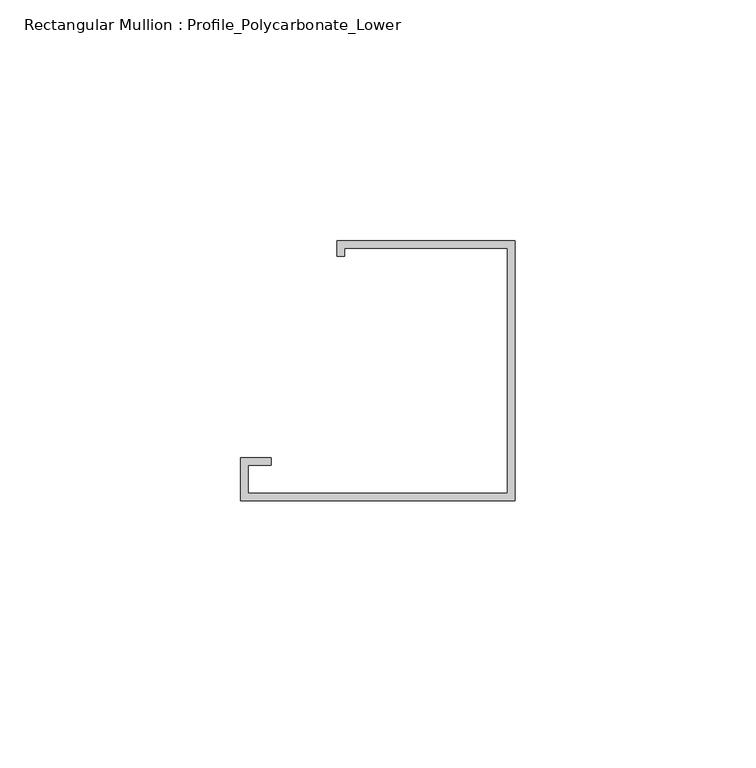
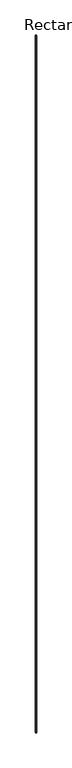
"""IFC4 building model written with IfcOpenShell, lengths in millimetres: member geometry, Rectangular Mullion : Profile_Polycarbonate_Lower."""

from ifc_helpers import new_model, si_unit, frame, origin, place, context, project, spatial, polyline, outline, extrude, source, transform, mapped, element, save


def rectangular_mullion_profile_polycarbonate_lower_9942ed0a(model_context):
    return source(origin(), model_context, "Body", "SweptSolid", [
        extrude(outline(polyline([(0.0, -28.984575), (-56.9976, -28.984575), (-56.9976, -19.992975), (-50.6476, -19.992975), (-50.6476, -21.580475), (-55.4101, -21.580475), (-55.4101, -27.397075), (-1.5875, -27.397075), (-1.5875, 23.428325), (-35.3949, 23.428325), (-35.3949, 21.840825), (-36.9824, 21.840825), (-36.9824, 25.015825), (0.0, 25.015825), (0.0, -28.984575)])), frame((0.0, 0.0, -31440.30288), z_axis=(0.0, 0.0, 1.0), x_axis=(1.0, 0.0, 0.0)), (0.0, 0.0, 1.0), 31440.30288),
    ])


if __name__ == "__main__":
    model = new_model("IFC4")
    model_context = context("Model", 3, world=origin())
    ifc_project = project(units=[si_unit("LENGTHUNIT", "METRE", prefix="MILLI")], contexts=[model_context])
    site = spatial("IfcSite", under=ifc_project)
    building = spatial("IfcBuilding", under=site)
    placement = place(None, origin())
    rectangular_mullion_profile_polycarbonate_lower_shape = rectangular_mullion_profile_polycarbonate_lower_9942ed0a(model_context)
    element("IfcMember", 1, ObjectType="Rectangular Mullion : Profile_Polycarbonate_Lower", at=placement, inside=building, context=model_context, shape_type="MappedRepresentation", body=[
        mapped(rectangular_mullion_profile_polycarbonate_lower_shape, transform((0.0, 0.0, 0.0), x_axis=(1.0, 0.0, 0.0), y_axis=(0.0, 1.0, 0.0), z_axis=(0.0, 0.0, 1.0))),
    ])
    save(model, "model.ifc")

# Revit data of these elements
# Type "Rectangular Mullion : Profile_Polycarbonate_Lower"
#   built-in parameter 1007322 = 0.177167 (stored number, unit not read)
#   built-in parameter 1007321 = 0 (stored number, unit not read)
#   built-in parameter 1007320 = 0.00520833 (stored number, unit not read)
